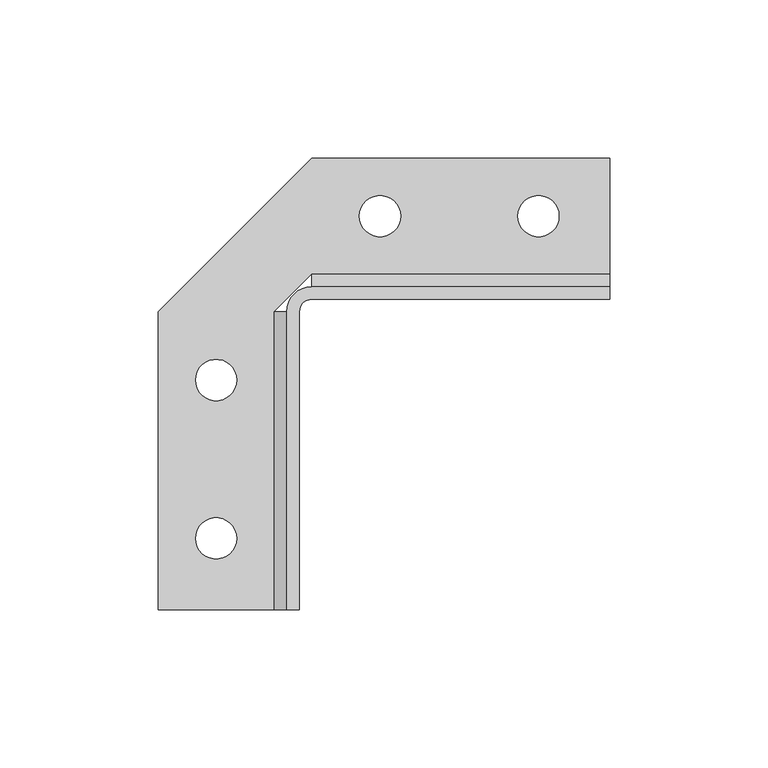
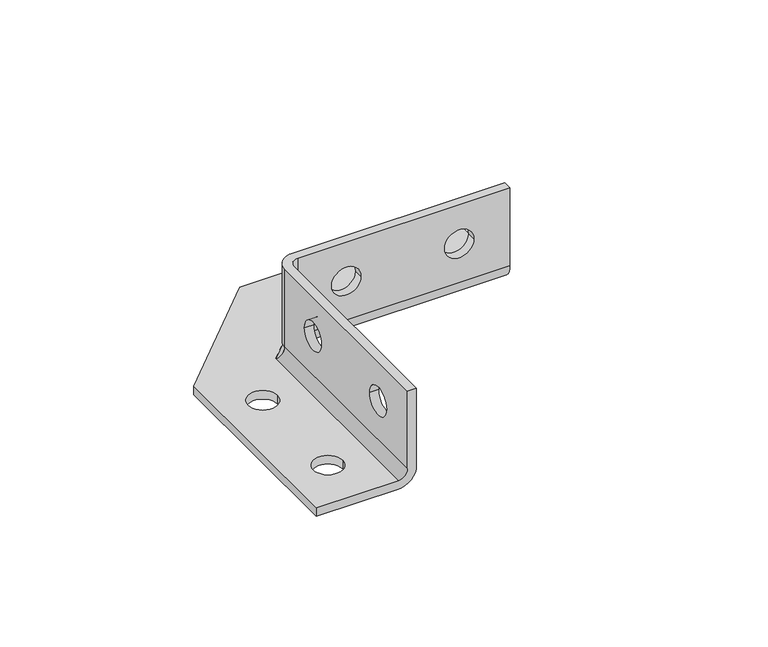
"""IFC4 building model written with IfcOpenShell, lengths in millimetres: proxy geometry, ➀ TN_Угол универсальный 90 (сборка тип 1) : ➀ TN_Угол универсальный 90 (сборка тип 1)."""

import ifcopenshell
import ifcopenshell.guid

model = None  # the IFC model being written
_history = None  # IfcOwnerHistory: only IFC2X3 demands one
_inside = {}  # id of a spatial element -> (the spatial element, [elements in it])
_under = {}  # id of a project, library or spatial element -> (it, [spatial elements below it])
_declared = {}  # id of a project -> (the project, [libraries it declares])
_typed = {}  # id of a type object -> (the type object, [elements of that type])
_made_of = {}  # id of a material, layer set ... -> (it, [elements and type objects made of it])


def new_model(schema):
    """Start an empty IFC model of exactly this schema.

    Asked for "IFC4X3", IfcOpenShell would pick the latest addendum, in which some entities
    have other attributes; the version numbers below select the first issue.
    IFC2X3 requires an IfcOwnerHistory on every rooted entity: one is made here for all.
    """
    global model, _history
    if schema == "IFC4X3":
        model = ifcopenshell.file(schema_version=(4, 3, 0, 0))
    else:
        model = ifcopenshell.file(schema=schema)
    _inside.clear()
    _under.clear()
    _declared.clear()
    _typed.clear()
    _made_of.clear()
    _history = None
    if model.schema == "IFC2X3":
        org = make("IfcOrganization", Name="unknown")
        user = make(
            "IfcPersonAndOrganization",
            ThePerson=make("IfcPerson", FamilyName="unknown"),
            TheOrganization=org,
        )
        app = make(
            "IfcApplication",
            ApplicationDeveloper=org,
            Version="unknown",
            ApplicationFullName="unknown",
            ApplicationIdentifier="unknown",
        )
        _history = make(
            "IfcOwnerHistory",
            OwningUser=user,
            OwningApplication=app,
            ChangeAction="ADDED",
            CreationDate=0,
        )
    return model


def make(cls, **values):
    """One entity of the class cls with the attributes given. An attribute that is None is left unset."""
    return model.create_entity(
        cls, **{name: value for name, value in values.items() if value is not None}
    )


def rooted(cls, **values):
    """An entity with a GlobalId (a new one), such as an element, a storey or a relation."""
    return make(cls, GlobalId=ifcopenshell.guid.new(), OwnerHistory=_history, **values)


def si_unit(unit_type, name, prefix=None):
    """IfcSIUnit, for example si_unit("LENGTHUNIT", "METRE", prefix="MILLI")."""
    return make("IfcSIUnit", UnitType=unit_type, Prefix=prefix, Name=name)


def assignment(units):
    """IfcUnitAssignment: the units of a project."""
    return None if units is None else make("IfcUnitAssignment", Units=units)


def point(xyz):
    """IfcCartesianPoint."""
    return None if xyz is None else make("IfcCartesianPoint", Coordinates=xyz)


def direction(xyz):
    """IfcDirection."""
    return None if xyz is None else make("IfcDirection", DirectionRatios=xyz)


def frame(location, z_axis=None, x_axis=None):
    """IfcAxis2Placement3D, a coordinate frame: its origin and axes. An axis left out is left unset."""
    return make(
        "IfcAxis2Placement3D",
        Location=point(location),
        Axis=direction(z_axis),
        RefDirection=direction(x_axis),
    )


def origin():
    """The frame at (0, 0, 0) with its axes left unset."""
    return frame((0.0, 0.0, 0.0))


def place(relative_to, where):
    """IfcLocalPlacement: puts the frame where relative to a parent placement (None: the world)."""
    return make(
        "IfcLocalPlacement", PlacementRelTo=relative_to, RelativePlacement=where
    )


def context(
    kind, dimensions, precision=None, world=None, true_north=None, identifier=None
):
    """IfcGeometricRepresentationContext, for example the 3D "Model" context."""
    return make(
        "IfcGeometricRepresentationContext",
        ContextIdentifier=identifier,
        ContextType=kind,
        CoordinateSpaceDimension=dimensions,
        Precision=precision,
        WorldCoordinateSystem=world,
        TrueNorth=true_north,
    )


def project(units=None, contexts=None):
    """IfcProject with its units and contexts."""
    return rooted(
        "IfcProject",
        Name="project",
        RepresentationContexts=contexts,
        UnitsInContext=assignment(units),
    )


def spatial(cls, under=None, at=None, **own):
    """A site, building, storey or space (cls), placed at a placement, below another one or the project."""
    s = rooted(cls, ObjectPlacement=at, **own)
    if under is not None:
        _under.setdefault(under.id(), (under, []))[1].append(s)
    return s


def polyline(points):
    """IfcPolyline through the points."""
    return make("IfcPolyline", Points=[point(p) for p in points])


def circle_curve(where, radius):
    """IfcCircle in the frame where."""
    return make("IfcCircle", Position=where, Radius=radius)


def shape(context_of_items, identifier, shape_type, items):
    """IfcShapeRepresentation: the items that make up one representation, for example the "Body"."""
    return make(
        "IfcShapeRepresentation",
        ContextOfItems=context_of_items,
        RepresentationIdentifier=identifier,
        RepresentationType=shape_type,
        Items=items,
    )


def source(mapping_origin, context_of_items, identifier, shape_type, items):
    """IfcRepresentationMap: a shape defined once, which mapped items show again and again."""
    return make(
        "IfcRepresentationMap",
        MappingOrigin=mapping_origin,
        MappedRepresentation=shape(context_of_items, identifier, shape_type, items),
    )


def transform(
    local_origin,
    x_axis=None,
    y_axis=None,
    z_axis=None,
    scale=None,
    scale2=None,
    scale3=None,
    uniform=True,
):
    """IfcCartesianTransformationOperator3D, or its non-uniform kind. x_axis, y_axis, z_axis: its Axis1, 2, 3."""
    if uniform:
        return make(
            "IfcCartesianTransformationOperator3D",
            Axis1=direction(x_axis),
            Axis2=direction(y_axis),
            LocalOrigin=point(local_origin),
            Scale=scale,
            Axis3=direction(z_axis),
        )
    return make(
        "IfcCartesianTransformationOperator3DnonUniform",
        Axis1=direction(x_axis),
        Axis2=direction(y_axis),
        LocalOrigin=point(local_origin),
        Scale=scale,
        Axis3=direction(z_axis),
        Scale2=scale2,
        Scale3=scale3,
    )


def mapped(mapping_source, mapping_target):
    """IfcMappedItem: shows the shape of a source again, moved by a transform."""
    return make(
        "IfcMappedItem", MappingSource=mapping_source, MappingTarget=mapping_target
    )


def made_of(thing, what):
    """Note that an element or type object is made of a material, layer set ...; save() writes the relation."""
    if what is not None:
        _made_of.setdefault(what.id(), (what, []))[1].append(thing)
    return thing


def element(
    cls,
    number,
    at=None,
    inside=None,
    cuts=None,
    type_object=None,
    material=None,
    context=None,
    identifier="Body",
    shape_type=None,
    held_by="IfcProductDefinitionShape",
    body=None,
    shapes=None,
    **own,
):
    """One element of the class cls, such as IfcWall. Its Tag is "e" and its number.

    at: its placement. inside: the storey or other place that contains it. cuts: it is an
    opening in that element (IfcRelVoidsElement). A single representation is given by context,
    identifier, shape_type and body (its items); several are given by shapes. held_by: the class
    of the entity that holds the representations. save() writes the other relations.
    """
    e = rooted(cls, Tag="e%d" % number, ObjectPlacement=at, **own)
    if body is not None:
        shapes = [shape(context, identifier, shape_type, body)]
    if shapes is not None:
        e.Representation = make(held_by, Representations=shapes)
    if inside is not None:
        _inside.setdefault(inside.id(), (inside, []))[1].append(e)
    if cuts is not None:
        rooted(
            "IfcRelVoidsElement", RelatingBuildingElement=cuts, RelatedOpeningElement=e
        )
    if type_object is not None:
        _typed.setdefault(type_object.id(), (type_object, []))[1].append(e)
    return made_of(e, material)


def aggregate(whole, parts):
    """IfcRelAggregates: a whole, such as a stair, and the parts it consists of."""
    return rooted("IfcRelAggregates", RelatingObject=whole, RelatedObjects=parts)


def save(model, path):
    """Write the relations noted so far, then the file.

    IfcRelAggregates (storeys below a building ...), IfcRelContainedInSpatialStructure (elements
    in a storey), IfcRelDefinesByType, IfcRelAssociatesMaterial and IfcRelDeclares: one each for
    every whole, place, type object, material and project.
    """
    for whole, parts in _under.values():
        aggregate(whole, parts)
    for where, things in _inside.values():
        rooted(
            "IfcRelContainedInSpatialStructure",
            RelatedElements=things,
            RelatingStructure=where,
        )
    for kind, things in _typed.values():
        rooted("IfcRelDefinesByType", RelatedObjects=things, RelatingType=kind)
    for what, things in _made_of.values():
        rooted("IfcRelAssociatesMaterial", RelatedObjects=things, RelatingMaterial=what)
    for by, libraries in _declared.values():
        rooted("IfcRelDeclares", RelatingContext=by, RelatedDefinitions=libraries)
    model.write(path)


def plane_surface(at):
    """IfcPlane: the flat surface through the origin of the frame at, square to its z axis."""
    return make("IfcPlane", Position=at)


def cylinder_surface(at, radius):
    """IfcCylindricalSurface: all points at the distance radius from the z axis of the frame at."""
    return make("IfcCylindricalSurface", Position=at, Radius=radius)


def revolved_surface(curve, axis_point, axis_direction):
    """IfcSurfaceOfRevolution: the curve turned about the line through axis_point along axis_direction."""
    return make(
        "IfcSurfaceOfRevolution",
        SweptCurve=make("IfcArbitraryOpenProfileDef", ProfileType="CURVE", Curve=curve),
        AxisPosition=make("IfcAxis1Placement", Location=point(axis_point), Axis=direction(axis_direction)),
    )


def advanced_brep(points, edges, surfaces, faces):
    """IfcAdvancedBrep: a solid bounded by faces that lie on surfaces and meet in shared edges.

    An edge is (start, end): straight between two places in points (the first is 0);
    or (start, end, curve); or (start, end, curve, False) where it runs against its curve.
    A face is (place in surfaces, loops), or (place, loops, False) where it looks against
    its surface's normal. A loop lists edges by number (the first is 1), with a minus sign
    where the edge is run from its end to its start. The first loop is the outer one.
    """
    corners = [point(p) for p in points]
    vertices = [make("IfcVertexPoint", VertexGeometry=c) for c in corners]
    made = []
    for start, end, *more in edges:
        made.append(
            make(
                "IfcEdgeCurve",
                EdgeStart=vertices[start],
                EdgeEnd=vertices[end],
                EdgeGeometry=more[0] if more else make("IfcPolyline", Points=[corners[start], corners[end]]),
                SameSense=more[1] if len(more) > 1 else True,
            )
        )
    hull = []
    for where, loops, *sense in faces:
        bounds = []
        for j, loop in enumerate(loops):
            ring = [make("IfcOrientedEdge", EdgeElement=made[abs(k) - 1], Orientation=k > 0) for k in loop]
            bounds.append(
                make(
                    "IfcFaceOuterBound" if j == 0 else "IfcFaceBound",
                    Bound=make("IfcEdgeLoop", EdgeList=ring),
                    Orientation=True,
                )
            )
        hull.append(make("IfcAdvancedFace", Bounds=bounds, FaceSurface=surfaces[where], SameSense=sense[0] if sense else True))
    return make("IfcAdvancedBrep", Outer=make("IfcClosedShell", CfsFaces=hull))


def generic_models_261a8f01(model_context):
    return source(origin(), model_context, "Body", "AdvancedBrep", [
        advanced_brep(
        [(-48.5, -94.0, 4.0), (-12.0, -94.0, 4.0), (-12.0, 0.0, 4.0), (0.0, 12.0, 4.0), (94.0, 12.0, 4.0), (94.0, 48.5, 4.0), (0.0, 48.5, 4.0), (-48.5, 0.0, 4.0), (-36.75, -71.5, 4.0), (-23.75, -71.5, 4.0), (-36.75, -21.5, 4.0), (-23.75, -21.5, 4.0), (65.0, 30.25, 4.0), (78.0, 30.25, 4.0), (15.0, 30.25, 4.0), (28.0, 30.25, 4.0), (-48.5, -94.0, 0.0), (-48.5, 0.0, 0.0), (0.0, 48.5, 0.0), (94.0, 48.5, 0.0), (94.0, 12.0, 0.0), (0.0, 12.0, 0.0), (-12.0, 0.0, 0.0), (-12.0, -94.0, 0.0), (-36.75, -71.5, 0.0), (-23.75, -71.5, 0.0), (-36.75, -21.5, 0.0), (-23.75, -21.5, 0.0), (65.0, 30.25, 0.0), (78.0, 30.25, 0.0), (15.0, 30.25, 0.0), (28.0, 30.25, 0.0), (0.0, 4.0, 8.0), (0.0, 8.0, 8.0), (94.0, 8.0, 8.0), (94.0, 4.0, 8.0), (-4.0, 0.0, 8.0), (-8.0, 0.0, 8.0), (-8.0, -94.0, 8.0), (-4.0, -94.0, 8.0), (-4.0, -94.0, 44.5), (-8.0, -94.0, 44.5), (-4.0, 0.0, 44.5), (-4.0, -78.0, 26.25), (-4.0, -65.0, 26.25), (-4.0, -28.0, 26.25), (-4.0, -15.0, 26.25), (0.0, 4.0, 44.5), (94.0, 4.0, 44.5), (94.0, 8.0, 44.5), (0.0, 8.0, 44.5), (-8.0, 0.0, 44.5), (-8.0, -65.0, 26.25), (-8.0, -78.0, 26.25), (-8.0, -15.0, 26.25), (-8.0, -28.0, 26.25), (65.0, 4.0, 26.25), (78.0, 4.0, 26.25), (15.0, 4.0, 26.25), (28.0, 4.0, 26.25), (78.0, 8.0, 26.25), (65.0, 8.0, 26.25), (28.0, 8.0, 26.25), (15.0, 8.0, 26.25)],
        [
            (0, 1),
            (1, 2),
            (2, 3),
            (3, 4),
            (4, 5),
            (5, 6),
            (6, 7),
            (7, 0),
            (8, 9, circle_curve(frame((-30.25, -71.5, 4.0), z_axis=(0.0, 0.0, -1.0), x_axis=(1.0, 0.0, 0.0)), 6.5)),
            (9, 8, circle_curve(frame((-30.25, -71.5, 4.0), z_axis=(0.0, 0.0, -1.0), x_axis=(1.0, 0.0, 0.0)), 6.5)),
            (10, 11, circle_curve(frame((-30.25, -21.5, 4.0), z_axis=(0.0, 0.0, -1.0), x_axis=(1.0, 0.0, 0.0)), 6.5)),
            (11, 10, circle_curve(frame((-30.25, -21.5, 4.0), z_axis=(0.0, 0.0, -1.0), x_axis=(1.0, 0.0, 0.0)), 6.5)),
            (12, 13, circle_curve(frame((71.5, 30.25, 4.0), z_axis=(0.0, 0.0, -1.0), x_axis=(1.0, 0.0, 0.0)), 6.5)),
            (13, 12, circle_curve(frame((71.5, 30.25, 4.0), z_axis=(0.0, 0.0, -1.0), x_axis=(1.0, 0.0, 0.0)), 6.5)),
            (14, 15, circle_curve(frame((21.5, 30.25, 4.0), z_axis=(0.0, 0.0, -1.0), x_axis=(1.0, 0.0, 0.0)), 6.5)),
            (15, 14, circle_curve(frame((21.5, 30.25, 4.0), z_axis=(0.0, 0.0, -1.0), x_axis=(1.0, 0.0, 0.0)), 6.5)),
            (16, 17),
            (17, 18),
            (18, 19),
            (19, 20),
            (20, 21),
            (21, 22),
            (22, 23),
            (23, 16),
            (24, 25, circle_curve(frame((-30.25, -71.5, 0.0), z_axis=(0.0, 0.0, 1.0), x_axis=(1.0, 0.0, 0.0)), 6.5)),
            (25, 24, circle_curve(frame((-30.25, -71.5, 0.0), z_axis=(0.0, 0.0, 1.0), x_axis=(1.0, 0.0, 0.0)), 6.5)),
            (26, 27, circle_curve(frame((-30.25, -21.5, 0.0), z_axis=(0.0, 0.0, 1.0), x_axis=(1.0, 0.0, 0.0)), 6.5)),
            (27, 26, circle_curve(frame((-30.25, -21.5, 0.0), z_axis=(0.0, 0.0, 1.0), x_axis=(1.0, 0.0, 0.0)), 6.5)),
            (28, 29, circle_curve(frame((71.5, 30.25, 0.0), z_axis=(0.0, 0.0, 1.0), x_axis=(1.0, 0.0, 0.0)), 6.5)),
            (29, 28, circle_curve(frame((71.5, 30.25, 0.0), z_axis=(0.0, 0.0, 1.0), x_axis=(1.0, 0.0, 0.0)), 6.5)),
            (30, 31, circle_curve(frame((21.5, 30.25, 0.0), z_axis=(0.0, 0.0, 1.0), x_axis=(1.0, 0.0, 0.0)), 6.5)),
            (31, 30, circle_curve(frame((21.5, 30.25, 0.0), z_axis=(0.0, 0.0, 1.0), x_axis=(1.0, 0.0, 0.0)), 6.5)),
            (2, 22),
            (21, 3),
            (5, 19),
            (18, 6),
            (17, 7),
            (16, 0),
            (8, 24),
            (25, 9),
            (10, 26),
            (27, 11),
            (12, 28),
            (29, 13),
            (14, 30),
            (31, 15),
            (21, 32, circle_curve(frame((0.0, 12.0, 8.0), z_axis=(-1.0, 0.0, 0.0), x_axis=(0.0, 1.0, 0.0)), 8.0)),
            (32, 33),
            (33, 3, circle_curve(frame((0.0, 12.0, 8.0), z_axis=(1.0, 0.0, 0.0), x_axis=(0.0, 1.0, 0.0)), 4.0)),
            (34, 4, circle_curve(frame((94.0, 12.0, 8.0), z_axis=(1.0, 0.0, 0.0), x_axis=(0.0, 1.0, 0.0)), 4.0)),
            (33, 34),
            (20, 35, circle_curve(frame((94.0, 12.0, 8.0), z_axis=(-1.0, 0.0, 0.0), x_axis=(0.0, 1.0, 0.0)), 8.0)),
            (35, 32),
            (36, 22, circle_curve(frame((-12.0, 0.0, 8.0), z_axis=(0.0, 1.0, 0.0), x_axis=(1.0, 0.0, 0.0)), 8.0)),
            (2, 37, circle_curve(frame((-12.0, 0.0, 8.0), z_axis=(0.0, -1.0, 0.0), x_axis=(1.0, 0.0, 0.0)), 4.0)),
            (37, 36),
            (1, 38, circle_curve(frame((-12.0, -94.0, 8.0), z_axis=(0.0, -1.0, 0.0), x_axis=(1.0, 0.0, 0.0)), 4.0)),
            (38, 37),
            (39, 23, circle_curve(frame((-12.0, -94.0, 8.0), z_axis=(0.0, 1.0, 0.0), x_axis=(1.0, 0.0, 0.0)), 8.0)),
            (36, 39),
            (39, 40),
            (40, 41),
            (41, 38),
            (36, 42),
            (42, 40),
            (43, 44, circle_curve(frame((-4.0, -71.5, 26.25), z_axis=(-1.0, 0.0, 0.0), x_axis=(0.0, -1.0, 0.0)), 6.5)),
            (44, 43, circle_curve(frame((-4.0, -71.5, 26.25), z_axis=(-1.0, 0.0, 0.0), x_axis=(0.0, -1.0, 0.0)), 6.5)),
            (45, 46, circle_curve(frame((-4.0, -21.5, 26.25), z_axis=(-1.0, 0.0, 0.0), x_axis=(0.0, -1.0, 0.0)), 6.5)),
            (46, 45, circle_curve(frame((-4.0, -21.5, 26.25), z_axis=(-1.0, 0.0, 0.0), x_axis=(0.0, -1.0, 0.0)), 6.5)),
            (42, 47, circle_curve(frame((0.0, 0.0, 44.5), z_axis=(0.0, 0.0, -1.0), x_axis=(-1.0, 0.0, 0.0)), 4.0)),
            (47, 48),
            (48, 49),
            (49, 50),
            (50, 51, circle_curve(frame((0.0, 0.0, 44.5), z_axis=(0.0, 0.0, 1.0), x_axis=(-1.0, 0.0, 0.0)), 8.0)),
            (51, 41),
            (51, 37),
            (52, 53, circle_curve(frame((-8.0, -71.5, 26.25), z_axis=(1.0, 0.0, 0.0), x_axis=(0.0, -1.0, 0.0)), 6.5)),
            (53, 52, circle_curve(frame((-8.0, -71.5, 26.25), z_axis=(1.0, 0.0, 0.0), x_axis=(0.0, -1.0, 0.0)), 6.5)),
            (54, 55, circle_curve(frame((-8.0, -21.5, 26.25), z_axis=(1.0, 0.0, 0.0), x_axis=(0.0, -1.0, 0.0)), 6.5)),
            (55, 54, circle_curve(frame((-8.0, -21.5, 26.25), z_axis=(1.0, 0.0, 0.0), x_axis=(0.0, -1.0, 0.0)), 6.5)),
            (37, 33, circle_curve(frame((0.0, 0.0, 8.0), z_axis=(0.0, 0.0, -1.0), x_axis=(-1.0, 0.0, 0.0)), 8.0)),
            (32, 36, circle_curve(frame((0.0, 0.0, 8.0), z_axis=(0.0, 0.0, 1.0), x_axis=(-1.0, 0.0, 0.0)), 4.0)),
            (32, 47),
            (50, 33),
            (48, 35),
            (34, 49),
            (56, 57, circle_curve(frame((71.5, 4.0, 26.25), z_axis=(0.0, 1.0, 0.0), x_axis=(-1.0, 0.0, 0.0)), 6.5)),
            (57, 56, circle_curve(frame((71.5, 4.0, 26.25), z_axis=(0.0, 1.0, 0.0), x_axis=(-1.0, 0.0, 0.0)), 6.5)),
            (58, 59, circle_curve(frame((21.5, 4.0, 26.25), z_axis=(0.0, 1.0, 0.0), x_axis=(-1.0, 0.0, 0.0)), 6.5)),
            (59, 58, circle_curve(frame((21.5, 4.0, 26.25), z_axis=(0.0, 1.0, 0.0), x_axis=(-1.0, 0.0, 0.0)), 6.5)),
            (60, 61, circle_curve(frame((71.5, 8.0, 26.25), z_axis=(0.0, -1.0, 0.0), x_axis=(-1.0, 0.0, 0.0)), 6.5)),
            (61, 60, circle_curve(frame((71.5, 8.0, 26.25), z_axis=(0.0, -1.0, 0.0), x_axis=(-1.0, 0.0, 0.0)), 6.5)),
            (62, 63, circle_curve(frame((21.5, 8.0, 26.25), z_axis=(0.0, -1.0, 0.0), x_axis=(-1.0, 0.0, 0.0)), 6.5)),
            (63, 62, circle_curve(frame((21.5, 8.0, 26.25), z_axis=(0.0, -1.0, 0.0), x_axis=(-1.0, 0.0, 0.0)), 6.5)),
            (56, 61),
            (60, 57),
            (58, 63),
            (62, 59),
            (43, 53),
            (52, 44),
            (45, 55),
            (54, 46),
        ],
        [
            plane_surface(frame((-48.5, -94.0, 4.0), z_axis=(0.0, 0.0, 1.0), x_axis=(1.0, 0.0, 0.0))),
            plane_surface(frame((-48.5, -94.0, 0.0), z_axis=(0.0, 0.0, -1.0), x_axis=(-1.0, 0.0, 0.0))),
            plane_surface(frame((-12.0, 0.0, 4.0), z_axis=(0.7071067811865553, -0.7071067811865398, 0.0), x_axis=(0.0, 0.0, -1.0))),
            plane_surface(frame((94.0, 48.5, 4.0), z_axis=(0.0, 1.0, 0.0), x_axis=(0.0, 0.0, -1.0))),
            plane_surface(frame((0.0, 48.5, 4.0), z_axis=(-0.7071067811865478, 0.7071067811865472, 0.0), x_axis=(0.0, 0.0, -1.0))),
            plane_surface(frame((-48.5, 0.0, 4.0), z_axis=(-1.0, 0.0, 0.0), x_axis=(0.0, 0.0, -1.0))),
            revolved_surface(polyline([(-23.75, -71.5, 0.0), (-23.75, -71.5, 4.0)]), (-30.25, -71.5, 0.0), (0.0, 0.0, -1.0)),
            revolved_surface(polyline([(-23.75, -21.5, 0.0), (-23.75, -21.5, 4.0)]), (-30.25, -21.5, 0.0), (0.0, 0.0, -1.0)),
            revolved_surface(polyline([(78.0, 30.25, 0.0), (78.0, 30.25, 4.0)]), (71.5, 30.25, 0.0), (0.0, 0.0, -1.0)),
            revolved_surface(polyline([(28.0, 30.25, 0.0), (28.0, 30.25, 4.0)]), (21.5, 30.25, 0.0), (0.0, 0.0, -1.0)),
            plane_surface(frame((0.0, 16.0, 8.0), z_axis=(-1.0, 0.0, 0.0), x_axis=(0.0, 0.0, 1.0))),
            revolved_surface(polyline([(0.0, 16.0, 8.0), (94.0, 16.0, 8.0)]), (0.0, 12.0, 8.0), (-1.0, 0.0, 0.0)),
            cylinder_surface(frame((0.0, 12.0, 8.0), z_axis=(1.0, 0.0, 0.0), x_axis=(0.0, 1.0, 0.0)), 8.0),
            plane_surface(frame((-8.0, 0.0, 8.0), z_axis=(0.0, 1.0, 0.0), x_axis=(1.0, 0.0, 0.0))),
            revolved_surface(polyline([(-8.0, 0.0, 8.0), (-8.0, -94.0, 8.0)]), (-12.0, 0.0, 8.0), (0.0, 1.0, 0.0)),
            cylinder_surface(frame((-12.0, 0.0, 8.0), z_axis=(0.0, -1.0, 0.0), x_axis=(1.0, 0.0, 0.0)), 8.0),
            plane_surface(frame((-4.0, -94.0, 8.0), z_axis=(0.0, -1.0, 0.0), x_axis=(0.0, 0.0, 1.0))),
            plane_surface(frame((-4.0, -94.0, 8.0), z_axis=(1.0, 0.0, 0.0), x_axis=(0.0, 1.0, 0.0))),
            plane_surface(frame((-4.0, -94.0, 44.5), z_axis=(0.0, 0.0, 1.0), x_axis=(0.0, 1.0, 0.0))),
            plane_surface(frame((-8.0, -94.0, 44.5), z_axis=(-1.0, 0.0, 0.0), x_axis=(0.0, 1.0, 0.0))),
            plane_surface(frame((-8.0, -94.0, 8.0), z_axis=(0.0, 0.0, -1.0), x_axis=(0.0, 1.0, 0.0))),
            revolved_surface(polyline([(-4.0, 0.0, 8.0), (-4.0, 0.0, 44.5)]), (0.0, 0.0, 8.0), (0.0, 0.0, -1.0)),
            cylinder_surface(frame((0.0, 0.0, 8.0), z_axis=(0.0, 0.0, -1.0), x_axis=(-1.0, 0.0, 0.0)), 8.0),
            plane_surface(frame((94.0, 4.0, 8.0), z_axis=(1.0, 0.0, 0.0), x_axis=(0.0, 0.0, 1.0))),
            plane_surface(frame((0.0, 4.0, 8.0), z_axis=(0.0, -1.0, 0.0), x_axis=(1.0, 0.0, 0.0))),
            plane_surface(frame((0.0, 8.0, 44.5), z_axis=(0.0, 1.0, 0.0), x_axis=(1.0, 0.0, 0.0))),
            revolved_surface(polyline([(65.0, 4.0, 26.25), (65.0, 8.0, 26.25)]), (71.5, 8.0, 26.25), (0.0, -1.0, 0.0)),
            revolved_surface(polyline([(15.0, 4.0, 26.25), (15.0, 8.0, 26.25)]), (21.5, 8.0, 26.25), (0.0, -1.0, 0.0)),
            revolved_surface(polyline([(-4.0, -78.0, 26.25), (-8.0, -78.0, 26.25)]), (-8.0, -71.5, 26.25), (1.0, 0.0, 0.0)),
            revolved_surface(polyline([(-4.0, -28.0, 26.25), (-8.0, -28.0, 26.25)]), (-8.0, -21.5, 26.25), (1.0, 0.0, 0.0)),
        ],
        [
            (0, [[1, 2, 3, 4, 5, 6, 7, 8], [9, 10], [11, 12], [13, 14], [15, 16]]),
            (1, [[17, 18, 19, 20, 21, 22, 23, 24], [25, 26], [27, 28], [29, 30], [31, 32]]),
            (2, [[-3, 33, -22, 34]]),
            (3, [[-6, 35, -19, 36]]),
            (4, [[-7, -36, -18, 37]]),
            (5, [[-8, -37, -17, 38]]),
            (6, [[-9, 39, -26, 40]]),
            (6, [[-10, -40, -25, -39]]),
            (7, [[-11, 41, -28, 42]]),
            (7, [[-12, -42, -27, -41]]),
            (8, [[-13, 43, -30, 44]]),
            (8, [[-14, -44, -29, -43]]),
            (9, [[-15, 45, -32, 46]]),
            (9, [[-16, -46, -31, -45]]),
            (10, [[47, 48, 49, -34]]),
            (11, [[50, -4, -49, 51]]),
            (12, [[52, 53, -47, -21]]),
            (13, [[54, -33, 55, 56]]),
            (14, [[57, 58, -55, -2]]),
            (15, [[59, -23, -54, 60]]),
            (16, [[61, 62, 63, -57, -1, -38, -24, -59]]),
            (17, [[-61, -60, 64, 65], [66, 67], [68, 69]]),
            (18, [[-62, -65, 70, 71, 72, 73, 74, 75]]),
            (19, [[-63, -75, 76, -58], [77, 78], [79, 80]]),
            (20, [[81, -48, 82, -56]]),
            (21, [[-64, -82, 83, -70]]),
            (22, [[-74, 84, -81, -76]]),
            (23, [[-72, 85, -52, -20, -35, -5, -50, 86]]),
            (24, [[-71, -83, -53, -85], [87, 88], [89, 90]]),
            (25, [[-73, -86, -51, -84], [91, 92], [93, 94]]),
            (26, [[95, -91, 96, -87]]),
            (26, [[-95, -88, -96, -92]]),
            (27, [[97, -93, 98, -89]]),
            (27, [[-97, -90, -98, -94]]),
            (28, [[99, -77, 100, -66]]),
            (28, [[-99, -67, -100, -78]]),
            (29, [[101, -79, 102, -68]]),
            (29, [[-101, -69, -102, -80]]),
        ],
    ),
    ])


if __name__ == "__main__":
    model = new_model("IFC4")
    model_context = context("Model", 3, world=origin())
    ifc_project = project(units=[si_unit("LENGTHUNIT", "METRE", prefix="MILLI")], contexts=[model_context])
    site = spatial("IfcSite", under=ifc_project)
    building = spatial("IfcBuilding", under=site)
    placement = place(None, origin())
    generic_models_shape = generic_models_261a8f01(model_context)
    element("IfcBuildingElementProxy", 1, Name="➀ TN_Угол универсальный 90 (сборка тип 1) : ➀ TN_Угол универсальный 90 (сборка тип 1)", ObjectType="➀ TN_Угол универсальный 90 (сборка тип 1) : ➀ TN_Угол универсальный 90 (сборка тип 1)", at=placement, inside=building, context=model_context, shape_type="MappedRepresentation", body=[
        mapped(generic_models_shape, transform((0.0, 0.0, 0.0), x_axis=(1.0, 0.0, 0.0), y_axis=(0.0, 1.0, 0.0), z_axis=(0.0, 0.0, 1.0))),
    ])
    save(model, "model.ifc")

# Revit data of these elements
# Type "➀ TN_Угол универсальный 90 (сборка тип 1) : ➀ TN_Угол универсальный 90 (сборка тип 1)"
#   Description = "Прочный универсальный угол предназначен для соединений элементов конструкций траверс, рамных и стеллажных систем. Угол обеспечивает усиление несущих конструкций для средних и тяжелых систем."
#   Manufacturer = "ТехноНИКОЛЬ"
#   Model = "Комплектующие к опорам"
#   URL = "https://nav.tn.ru/knowledge-base/polimernye-membrany/opory-pod-oborudovanie-na-ploskoy-krovle/?sphrase_id=266812"
#   ADSK_Обозначение = "ТехноНИКОЛЬ"
#   ADSK_Наименование краткое = "90° 38-41 4F8"
#   ADSK_Наименование = "Угол универсальный 90° 38-41 4F8"
#   ADSK_Масса_Текст = ""
#   ADSK_Марка = "90° 38-41 4F8"
#   ADSK_Код изделия = "660820"
#   ADSK_Завод-изготовитель = "ТехноНИКОЛЬ"
#   ADSK_Единица измерения = "шт."
#   ADSK_Группирование = "Комплектующие к опорам"
#   ADSK_URL страницы изделия = "https://nav.tn.ru/knowledge-base/polimernye-membrany/opory-pod-oborudovanie-na-ploskoy-krovle/?sphrase_id=266812"
#   ADSK_URL документации изделия = ""
#   Размер_Толщина = 4 mm
#   ADSK_Количество = 1
#   ADSK_Материал = TN_СтальГальванизированная_Серый
#   Default Elevation = 0
# Element 1 (IfcBuildingElementProxy, "➀ TN_Угол универсальный 90 (сборка тип 1) : ➀ TN_Угол универсальный 90 (сборка тип 1)")
#   Materials on its faces: "TN_СтальГальванизированная_Серый"
# Materials
#   "TN_СтальГальванизированная_Серый": class "Типовые", colour RGB 206 210 213, transparency 0, Cost = 0
